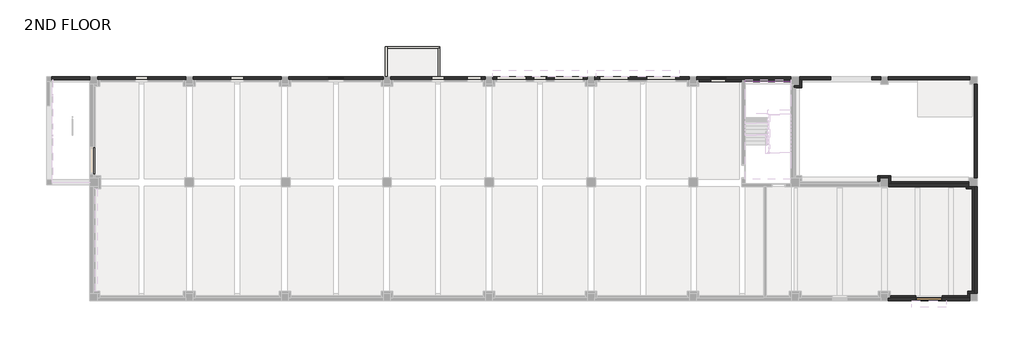
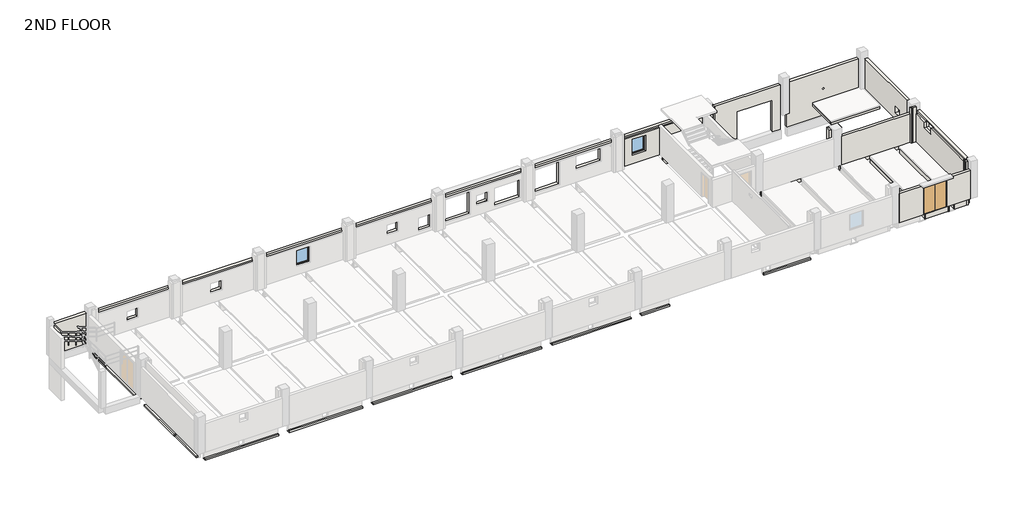
# One storey, part 3 of 7: 46 walls, 2 slabs, 2 windows, 1 door.
# Revit data of these elements (continued)
# Type "Double Door_Steel : H_DR_AR B12_Door_Double_W2100xH2580_No FR_SD-5"
#   Type Mark = "444"
#   프레임 = ""
#   철물 = ""
#   유리/마감 = ""
#   위치/개소 = ""
#   부호 = ""
#   문번호 = ""
#   문기호 = "SD-5"
#   Analytic Construction = "<None>"
#   Door Width = 1005 mm
#   Height = 2580 mm
#   Width = 2100 mm
#   Define Thermal Properties by = 1
#   문 틀 = none
#   문 = none
#   Function = (empty or 0)
#   Assembly Code = ""
#   Wall Closure = (empty or 0)
# Type "H_WA_AR_B02_Int Wall_2L Gypsum_Insulationl_T154(Mirror)"
#   Keynote = ""
#   Type Comments = ""
#   Description = ""
#   Function = 0
#   Layers, outside or top first: 135 mm "00_Insulation_Glass Wool" (function 1); 9.5 mm "00_Finish_Gypsum Board" (function 4); 9.5 mm "00_Finish_Gypsum Board" (function 4)
# Type "H_WA_AR B02_Ext Wall RC-AG_T250_W1"
#   Type Comments = "CV-AG"
#   H_Rebar Ratio = 0.12
#   Layers, outside or top first: 250 mm "Concrete_f'c=28MPa(Cylender)" (function 1)
# Type "H_WA_AR B02_Int Wall RC-AG_T250_W2"
#   Type Comments = "CV-AG"
#   H_Rebar Ratio = 0.12
#   Layers, outside or top first: 250 mm "Concrete_f'c=28MPa(Cylender)" (function 1)
# Type "H_WA_AR B02_Ext Wall RC-AG_T150"
#   Type Comments = "CV-AG"
#   H_Rebar Ratio = 0.12
#   Layers, outside or top first: 150 mm "Concrete_f'c=28MPa(Cylender)" (function 1)
# Type "H_WA_AR_B02_Ext Wall_Concrete Lintel_T190"
#   Type Comments = "CV-AG"
#   H_Rebar Ratio = 0.12
#   Layers, outside or top first: 190 mm "00_Concrete_Plain Conc." (function 1)
# Type "H_WA_AR B02_Ext Wall DY-IN_T154"
#   Type Comments = ""
#   Layers, outside or top first: 0 mm "00_Finish_Paint_Vinyl Paint" (function 100); 9.5 mm "00_Finish_Gypsum Board" (function 4); 9.5 mm "00_Finish_Gypsum Board" (function 4); 135 mm "00_Insulation_Glass Wool" (function 3); 0 mm no material (function 100)
# Type "H_CE_AR_B09_Souns Absorbing_100T_C7"
#   Type Comments = "finish"
#   Layers, outside or top first: 100 mm "00.Ceiling_Sound Absorbing" (function 4)
# Type "H_CE_AR_B09_Souns Absorbing_100T_C7 2"
#   Type Comments = "finish"
#   Layers, outside or top first: 164 mm "00.Ceiling_Sound Absorbing" (function 4)
# Type "Fixed Window : H_WD_AR_B11_Fix_Steel Window_SG_W1200xH1500_AW-2"
#   Type Mark = "269"
#   Analytic Construction = "<None>"
#   창 두께 = 150 mm
#   Height = 1500 mm
#   절반 창 두께 = 75 mm
#   기본 씰 높이 = 800 mm
#   Width = 1200 mm
#   ▽ = yes
#   Define Thermal Properties by = 1
#   창 패널 = none
#   창 프레임 = none
#   Wall Closure = (empty or 0)
#   Description = (empty or 0)
# Element 1 (IfcDoor, "Double Door_Steel : H_DR_AR B12_Door_Double_W2100xH2580_No FR_SD-5")
#   Phase Created = New Construction
# Element 2 (IfcSlab, "H_WA_AR_B02_Int Wall_2L Gypsum_Insulationl_T154(Mirror)")
#   Height Offset From Level = -710 mm
#   Phase Created = New Construction
#   Materials on its faces: "00_Finish_Gypsum Board", "00_Insulation_Glass Wool"
# Element 3 (IfcSlab, "H_WA_AR_B02_Int Wall_2L Gypsum_Insulationl_T154(Mirror)")
#   built-in parameter 1001955 = 1.5708 (stored number, unit not read)
#   Height Offset From Level = -810 mm
#   Phase Created = New Construction
#   Materials on its faces: "00_Finish_Gypsum Board", "00_Insulation_Glass Wool"
# Elements 4, 5, 6, 7, 8, 9, 10, 15 (IfcWall, "H_WA_AR B02_Ext Wall RC-AG_T250_W1")
#   Comments = ""
#   Top Offset = -800 mm
#   Base Offset = 0 mm
#   wall height = 2700 mm
#   Phase Created = New Construction
#   Base Constraint = 2ND FLOOR
#   Top Constraint = 3RD FLOOR
#   Materials on its faces: "Concrete_f'c=28MPa(Cylender)"
# Elements 11, 12 (IfcWall, "H_WA_AR B02_Ext Wall RC-AG_T250_W1")
#   Comments = ""
#   built-in parameter 1001111 = -1500 mm
#   Top Offset = -800 mm
#   Base Offset = -1500 mm
#   wall height = 4200 mm
#   Phase Created = New Construction
#   Base Constraint = 2ND FLOOR
#   Top Constraint = 3RD FLOOR
#   Materials on its faces: "Concrete_f'c=28MPa(Cylender)"
# Elements 13, 14 (IfcWall, "H_WA_AR B02_Ext Wall RC-AG_T250_W1")
#   Comments = ""
#   Top Offset = -700 mm
#   Base Offset = 0 mm
#   wall height = 2800 mm
#   Phase Created = New Construction
#   Base Constraint = 2ND FLOOR
#   Top Constraint = 3RD FLOOR
#   Materials on its faces: "Concrete_f'c=28MPa(Cylender)"
# Element 16 (IfcWall, "H_WA_AR B02_Ext Wall RC-AG_T250_W1")
#   Comments = ""
#   built-in parameter 1001111 = -50 mm
#   Top Offset = -650 mm
#   Base Offset = -50 mm
#   wall height = 2900 mm
#   Phase Created = New Construction
#   Base Constraint = 2ND FLOOR
#   Top Constraint = 3RD FLOOR
#   Materials on its faces: "Concrete_f'c=28MPa(Cylender)"
# Element 17 (IfcWall, "H_WA_AR B02_Int Wall RC-AG_T250_W2")
#   Comments = ""
#   Top Offset = -800 mm
#   Base Offset = 0 mm
#   wall height = 2700 mm
#   Phase Created = New Construction
#   Base Constraint = 2ND FLOOR
#   Top Constraint = 3RD FLOOR
#   Materials on its faces: "Concrete_f'c=28MPa(Cylender)"
# Elements 18, 19, 20 (IfcWall, "H_WA_AR B02_Ext Wall RC-AG_T150")
#   Comments = ""
#   built-in parameter 1001111 = -1300 mm
#   Top Offset = -700 mm
#   Base Offset = -1300 mm
#   wall height = 600 mm
#   Phase Created = New Construction
#   Base Constraint = 2ND FLOOR
#   Top Constraint = 2ND FLOOR
#   Materials on its faces: "Concrete_f'c=28MPa(Cylender)"
# Elements 21, 22 (IfcWall, "H_WA_AR_B02_Ext Wall_Concrete Lintel_T190")
#   Comments = ""
#   built-in parameter 1001111 = -340 mm
#   Top Offset = -150 mm
#   Base Offset = -340 mm
#   wall height = 190 mm
#   Phase Created = New Construction
#   Base Constraint = 2ND FLOOR
#   Top Constraint = 2ND FLOOR
#   Materials on its faces: "00_Concrete_Plain Conc."
# Element 23 (IfcWall, "H_WA_AR B02_Ext Wall DY-IN_T154")
#   Top Offset = -945 mm
#   Base Offset = 0 mm
#   wall height = 2555 mm
#   Phase Created = New Construction
#   Base Constraint = 2ND FLOOR
#   Top Constraint = 3RD FLOOR
#   Materials on its faces: "Default Wall", "00_Insulation_Glass Wool", "00_Finish_Gypsum Board"
# Element 24 (IfcWall, "H_WA_AR B02_Ext Wall DY-IN_T154")
#   Top Offset = -845 mm
#   Base Offset = 0 mm
#   wall height = 2655 mm
#   Phase Created = New Construction
#   Base Constraint = 2ND FLOOR
#   Top Constraint = 3RD FLOOR
#   Materials on its faces: "Default Wall", "00_Insulation_Glass Wool", "00_Finish_Gypsum Board"
# Element 25 (IfcWall, "H_WA_AR B02_Ext Wall DY-IN_T154")
#   Top Offset = -180 mm
#   Base Offset = 0 mm
#   wall height = 3320 mm
#   Phase Created = New Construction
#   Base Constraint = 2ND FLOOR
#   Top Constraint = 3RD FLOOR
#   Materials on its faces: "00_Insulation_Glass Wool", "Default Wall", "00_Finish_Gypsum Board"
# Elements 26, 27, 33 (IfcWall, "H_WA_AR B02_Ext Wall DY-IN_T154")
#   Top Offset = -180 mm
#   Base Offset = 0 mm
#   wall height = 3320 mm
#   Phase Created = New Construction
#   Base Constraint = 2ND FLOOR
#   Top Constraint = 3RD FLOOR
#   Materials on its faces: "Default Wall", "00_Insulation_Glass Wool", "00_Finish_Gypsum Board"
# Elements 28, 32 (IfcWall, "H_WA_AR B02_Ext Wall DY-IN_T154")
#   Top Offset = -180 mm
#   Base Offset = 0 mm
#   wall height = 3320 mm
#   Phase Created = New Construction
#   Base Constraint = 2ND FLOOR
#   Top Constraint = 3RD FLOOR
#   Materials on its faces: "Default Wall", "00_Finish_Gypsum Board", "00_Insulation_Glass Wool"
# Element 29 (IfcWall, "H_WA_AR B02_Ext Wall DY-IN_T154")
#   Top Offset = -945 mm
#   Base Offset = 0 mm
#   wall height = 2555 mm
#   Phase Created = New Construction
#   Base Constraint = 2ND FLOOR
#   Top Constraint = 3RD FLOOR
#   Materials on its faces: "Default Wall", "00_Finish_Gypsum Board", "00_Insulation_Glass Wool"
# Element 30 (IfcWall, "H_WA_AR B02_Ext Wall DY-IN_T154")
#   Top Offset = -334 mm
#   Base Offset = 0 mm
#   wall height = 3166 mm
#   Phase Created = New Construction
#   Base Constraint = 2ND FLOOR
#   Top Constraint = 3RD FLOOR
#   Materials on its faces: "Default Wall", "00_Finish_Gypsum Board", "00_Insulation_Glass Wool"
# Element 31 (IfcWall, "H_WA_AR B02_Ext Wall DY-IN_T154")
#   Top Offset = -334 mm
#   Base Offset = 0 mm
#   wall height = 3166 mm
#   Phase Created = New Construction
#   Base Constraint = 2ND FLOOR
#   Top Constraint = 3RD FLOOR
#   Materials on its faces: "Default Wall", "00_Insulation_Glass Wool", "00_Finish_Gypsum Board"
# Element 34 (IfcWall, "H_WA_AR B02_Ext Wall DY-IN_T154")
#   Top Offset = -180 mm
#   Base Offset = 0 mm
#   wall height = 3320 mm
#   Phase Created = New Construction
#   Base Constraint = 2ND FLOOR
#   Top Constraint = 3RD FLOOR
#   Materials on its faces: "00_Insulation_Glass Wool", "00_Finish_Gypsum Board", "Default Wall"
# Element 35 (IfcWall, "H_WA_AR B02_Ext Wall DY-IN_T154")
#   built-in parameter 1001111 = 135 mm
#   Top Offset = -945 mm
#   Base Offset = 135 mm
#   wall height = 2420 mm
#   Phase Created = New Construction
#   Base Constraint = 2ND FLOOR
#   Top Constraint = 3RD FLOOR
#   Materials on its faces: "Default Wall", "00_Insulation_Glass Wool", "00_Finish_Gypsum Board"
# Elements 36, 37 (IfcWall, "H_WA_AR B02_Ext Wall DY-IN_T154")
#   built-in parameter 1001111 = -935 mm
#   Top Offset = 135 mm
#   Base Offset = -935 mm
#   wall height = 1070 mm
#   Phase Created = New Construction
#   Base Constraint = 2ND FLOOR
#   Top Constraint = 2ND FLOOR
#   Materials on its faces: "Default Wall", "00_Insulation_Glass Wool", "00_Finish_Gypsum Board"
# Element 38 (IfcWall, "H_WA_AR B02_Ext Wall DY-IN_T154")
#   built-in parameter 1001111 = 135 mm
#   Top Offset = -2155 mm
#   Base Offset = 135 mm
#   wall height = 1210 mm
#   Phase Created = New Construction
#   Base Constraint = 2ND FLOOR
#   Top Constraint = 3RD FLOOR
#   Materials on its faces: "Default Wall", "00_Finish_Gypsum Board", "00_Insulation_Glass Wool"
# Element 39 (IfcWall, "H_WA_AR B02_Ext Wall DY-IN_T154")
#   built-in parameter 1001111 = -945 mm
#   Top Offset = 135 mm
#   Base Offset = -945 mm
#   wall height = 1080 mm
#   Phase Created = New Construction
#   Base Constraint = 2ND FLOOR
#   Top Constraint = 2ND FLOOR
#   Materials on its faces: "Default Wall", "00_Finish_Gypsum Board", "00_Insulation_Glass Wool"
# Element 40 (IfcWall, "H_WA_AR B02_Ext Wall DY-IN_T154")
#   built-in parameter 1001111 = 1545 mm
#   Top Offset = -945 mm
#   Base Offset = 1545 mm
#   wall height = 1010 mm
#   Phase Created = New Construction
#   Base Constraint = 2ND FLOOR
#   Top Constraint = 3RD FLOOR
#   Materials on its faces: "Default Wall", "00_Finish_Gypsum Board", "00_Insulation_Glass Wool"
# Elements 41, 42, 43, 44, 45, 46 (IfcWall, "H_CE_AR_B09_Souns Absorbing_100T_C7")
#   built-in parameter 1001111 = -800 mm
#   Top Offset = -250 mm
#   Base Offset = -800 mm
#   wall height = 550 mm
#   Phase Created = New Construction
#   Base Constraint = 2ND FLOOR
#   Top Constraint = 2ND FLOOR
#   Materials on its faces: "00.Ceiling_Sound Absorbing"
# Elements 47, 48 (IfcWall, "H_CE_AR_B09_Souns Absorbing_100T_C7 2")
#   built-in parameter 1001111 = -800 mm
#   Top Offset = -250 mm
#   Base Offset = -800 mm
#   wall height = 550 mm
#   Phase Created = New Construction
#   Base Constraint = 2ND FLOOR
#   Top Constraint = 2ND FLOOR
#   Materials on its faces: "00.Ceiling_Sound Absorbing"
# Element 49 (IfcWall, "H_CE_AR_B09_Souns Absorbing_100T_C7")
#   built-in parameter 1001111 = -700 mm
#   Top Offset = -250 mm
#   Base Offset = -700 mm
#   wall height = 450 mm
#   Phase Created = New Construction
#   Base Constraint = 2ND FLOOR
#   Top Constraint = 2ND FLOOR
#   Materials on its faces: "00.Ceiling_Sound Absorbing"
# Element 50 (IfcWindow, "Fixed Window : H_WD_AR_B11_Fix_Steel Window_SG_W1200xH1500_AW-2")
#   Mark = "FRW-13"
#   Phase Created = New Construction
#   Materials on its faces: "00_Metal_Aluminum", "Glass"
# Element 51 (IfcWindow, "Fixed Window : H_WD_AR_B11_Fix_Steel Window_SG_W1200xH1500_AW-2")
#   Mark = "FRW-14"
#   Phase Created = New Construction
#   Materials on its faces: "00_Metal_Aluminum", "Glass"
# Materials
#   "00_Insulation_Glass Wool": class "Insulation", colour RGB 200 200 140, transparency 0, Description = "Insulation(Loose)", Cost = 0
#   "00_Finish_Gypsum Board": class "Finish", colour RGB 171 170 168, transparency 0, Description = "Gypsum Board", Cost = 0, Image = Finishes.Gypsum Board.Painted.White.jpg
#   "Concrete_f'c=28MPa(Cylender)": class "Concrete", colour RGB 176 176 176, transparency 0, Description = "Reinf. Conc.", Cost = 0, Image = Concrete.Cast-In-Place.Flat.Polished.Grey.jpg
#   "00_Concrete_Plain Conc.": class "Concrete", colour RGB 176 176 176, transparency 0, Description = "Plain Conc.", Cost = 0, Image = Concrete.Cast-In-Place.Flat.Polished.Grey.jpg
#   "00_Finish_Paint_Vinyl Paint": class "Finish", colour RGB 128 128 64, transparency 0, Description = "Plastic", Cost = 0
#   "00.Ceiling_Sound Absorbing": class "Generic", colour RGB 100 102 90, transparency 0, Description = "Acoustic ceiling tile", Cost = 0
#   "Default Wall": class "Miscellaneous", colour RGB 80 80 80, transparency 0
#   "00_Metal_Aluminum": class "Metal", colour RGB 244 244 244, transparency 0, Description = "Aluminum", Cost = 0, Image = none
#   "Glass": class "Glass", colour RGB 218 227 224, transparency 0.85, Description = "Soda Lime Glass", Cost = 0
